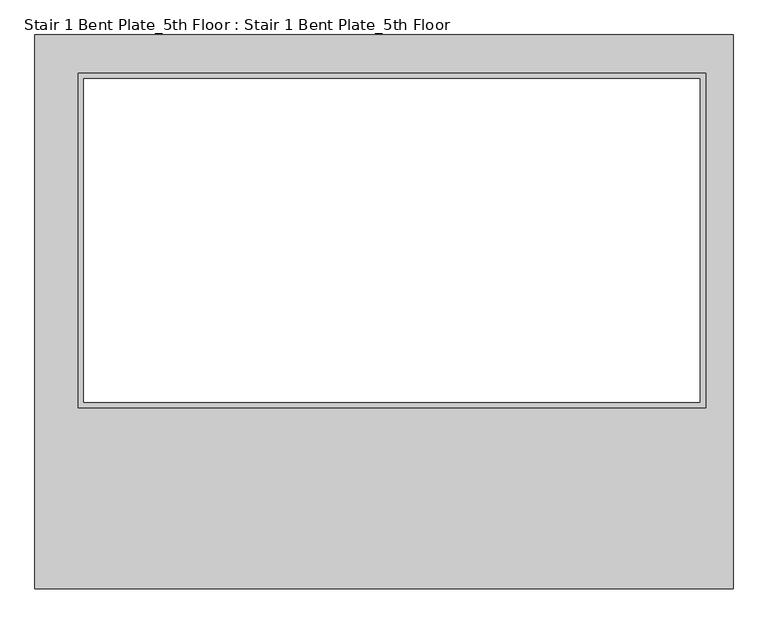
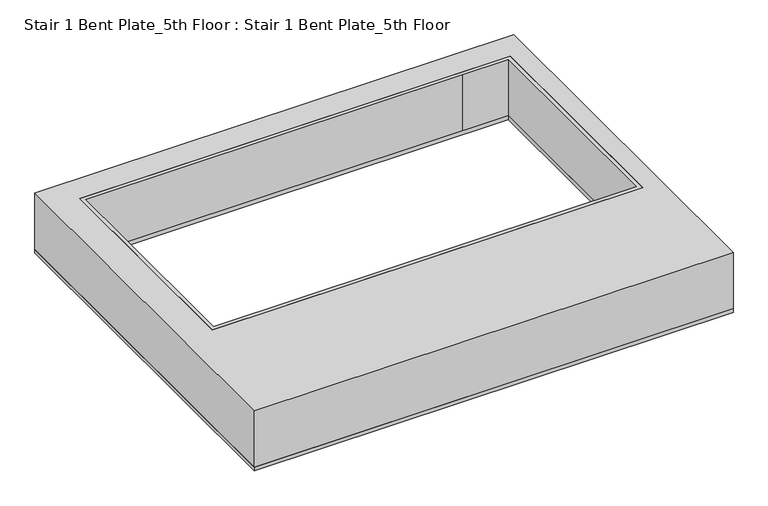
"""IFC4 building model written with IfcOpenShell, lengths in millimetres: proxy geometry, Stair 1 Bent Plate_5th Floor : Stair 1 Bent Plate_5th Floor."""

from ifc_helpers import new_model, si_unit, frame, origin, origin_with_axes, place, context, project, spatial, polyline, outline, extrude, source, transform, mapped, element, save


def stair_1_bent_plate_5th_floor_stair_1_bent_plate_5th_floor_5894586e(model_context):
    return source(origin(), model_context, "Body", "SweptSolid", [
        extrude(outline(polyline([(-342.9, -1112.8375), (-342.9, 106.3625), (1193.8, 106.3625), (1193.8, -1112.8375), (-342.9, -1112.8375)]), holes=[polyline([(1133.475, 22.225), (-247.65, 22.225), (-247.65, -714.375), (1133.475, -714.375), (1133.475, 22.225)])]), frame((0.0, 0.0, 12.7), z_axis=(0.0, 0.0, 1.0), x_axis=(1.0, 0.0, 0.0)), (0.0, 0.0, 1.0), 190.5),
        extrude(outline(polyline([(1193.8, -1112.8375), (-342.9, -1112.8375), (-342.9, 106.3625), (1193.8, 106.3625), (1193.8, -1112.8375)]), holes=[polyline([(-234.95, 9.525), (-234.95, -701.675), (1120.775, -701.675), (1120.775, 9.525), (-234.95, 9.525)])]), origin_with_axes(), (0.0, 0.0, 1.0), 12.7),
        extrude(outline(polyline([(1133.475, 22.225), (1133.475, -714.375), (-247.65, -714.375), (-247.65, 22.225), (1133.475, 22.225)]), holes=[polyline([(-234.95, -701.675), (1120.775, -701.675), (1120.775, 9.525), (974.725, 9.525), (-234.95, 9.525), (-234.95, -190.5), (-234.95, -701.675)])]), origin_with_axes(), (0.0, 0.0, 1.0), 203.2),
    ])


if __name__ == "__main__":
    model = new_model("IFC4")
    model_context = context("Model", 3, world=origin())
    ifc_project = project(units=[si_unit("LENGTHUNIT", "METRE", prefix="MILLI")], contexts=[model_context])
    site = spatial("IfcSite", under=ifc_project)
    building = spatial("IfcBuilding", under=site)
    placement = place(None, origin())
    stair_1_bent_plate_5th_floor_stair_1_bent_plate_5th_floor_shape = stair_1_bent_plate_5th_floor_stair_1_bent_plate_5th_floor_5894586e(model_context)
    element("IfcBuildingElementProxy", 1, Name="Stair 1 Bent Plate_5th Floor : Stair 1 Bent Plate_5th Floor", ObjectType="Stair 1 Bent Plate_5th Floor : Stair 1 Bent Plate_5th Floor", at=placement, inside=building, context=model_context, shape_type="MappedRepresentation", body=[
        mapped(stair_1_bent_plate_5th_floor_stair_1_bent_plate_5th_floor_shape, transform((0.0, 0.0, 0.0), x_axis=(1.0, 0.0, 0.0), y_axis=(0.0, 1.0, 0.0), z_axis=(0.0, 0.0, 1.0))),
    ])
    save(model, "model.ifc")

# Revit data of these elements
# Element 1 (IfcBuildingElementProxy, "Stair 1 Bent Plate_5th Floor : Stair 1 Bent Plate_5th Floor")
#   Materials on its faces: "Concrete Infill"
# Materials
#   "Concrete Infill": class "Generic", colour RGB 0 255 0, transparency 0, Cost = 0
